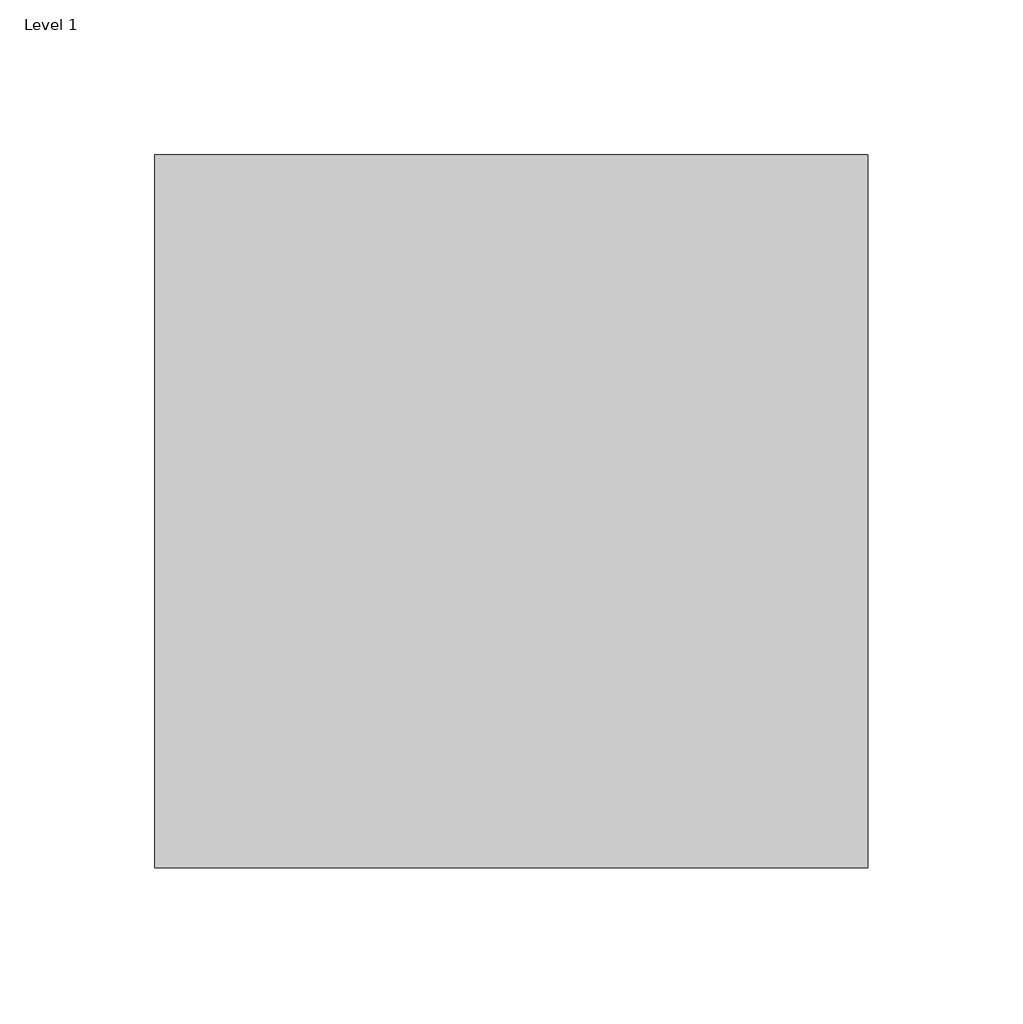
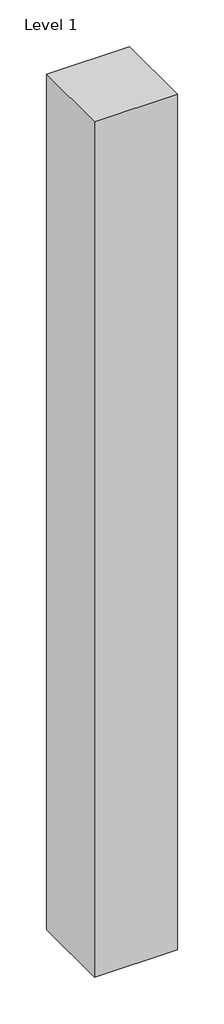
# One storey, part 1 of 2: 1 column.
"""IFC4 building model written with IfcOpenShell, lengths in millimetres."""

import ifcopenshell
import ifcopenshell.guid

model = None  # the IFC model being written
_history = None  # IfcOwnerHistory: only IFC2X3 demands one
_inside = {}  # id of a spatial element -> (the spatial element, [elements in it])
_under = {}  # id of a project, library or spatial element -> (it, [spatial elements below it])
_declared = {}  # id of a project -> (the project, [libraries it declares])
_typed = {}  # id of a type object -> (the type object, [elements of that type])
_made_of = {}  # id of a material, layer set ... -> (it, [elements and type objects made of it])


def new_model(schema):
    """Start an empty IFC model of exactly this schema.

    Asked for "IFC4X3", IfcOpenShell would pick the latest addendum, in which some entities
    have other attributes; the version numbers below select the first issue.
    IFC2X3 requires an IfcOwnerHistory on every rooted entity: one is made here for all.
    """
    global model, _history
    if schema == "IFC4X3":
        model = ifcopenshell.file(schema_version=(4, 3, 0, 0))
    else:
        model = ifcopenshell.file(schema=schema)
    _inside.clear()
    _under.clear()
    _declared.clear()
    _typed.clear()
    _made_of.clear()
    _history = None
    if model.schema == "IFC2X3":
        org = make("IfcOrganization", Name="unknown")
        user = make(
            "IfcPersonAndOrganization",
            ThePerson=make("IfcPerson", FamilyName="unknown"),
            TheOrganization=org,
        )
        app = make(
            "IfcApplication",
            ApplicationDeveloper=org,
            Version="unknown",
            ApplicationFullName="unknown",
            ApplicationIdentifier="unknown",
        )
        _history = make(
            "IfcOwnerHistory",
            OwningUser=user,
            OwningApplication=app,
            ChangeAction="ADDED",
            CreationDate=0,
        )
    return model


def make(cls, **values):
    """One entity of the class cls with the attributes given. An attribute that is None is left unset."""
    return model.create_entity(
        cls, **{name: value for name, value in values.items() if value is not None}
    )


def rooted(cls, **values):
    """An entity with a GlobalId (a new one), such as an element, a storey or a relation."""
    return make(cls, GlobalId=ifcopenshell.guid.new(), OwnerHistory=_history, **values)


def si_unit(unit_type, name, prefix=None):
    """IfcSIUnit, for example si_unit("LENGTHUNIT", "METRE", prefix="MILLI")."""
    return make("IfcSIUnit", UnitType=unit_type, Prefix=prefix, Name=name)


def assignment(units):
    """IfcUnitAssignment: the units of a project."""
    return None if units is None else make("IfcUnitAssignment", Units=units)


def point(xyz):
    """IfcCartesianPoint."""
    return None if xyz is None else make("IfcCartesianPoint", Coordinates=xyz)


def direction(xyz):
    """IfcDirection."""
    return None if xyz is None else make("IfcDirection", DirectionRatios=xyz)


def frame(location, z_axis=None, x_axis=None):
    """IfcAxis2Placement3D, a coordinate frame: its origin and axes. An axis left out is left unset."""
    return make(
        "IfcAxis2Placement3D",
        Location=point(location),
        Axis=direction(z_axis),
        RefDirection=direction(x_axis),
    )


def origin():
    """The frame at (0, 0, 0) with its axes left unset."""
    return frame((0.0, 0.0, 0.0))


def place(relative_to, where):
    """IfcLocalPlacement: puts the frame where relative to a parent placement (None: the world)."""
    return make(
        "IfcLocalPlacement", PlacementRelTo=relative_to, RelativePlacement=where
    )


def context(
    kind, dimensions, precision=None, world=None, true_north=None, identifier=None
):
    """IfcGeometricRepresentationContext, for example the 3D "Model" context."""
    return make(
        "IfcGeometricRepresentationContext",
        ContextIdentifier=identifier,
        ContextType=kind,
        CoordinateSpaceDimension=dimensions,
        Precision=precision,
        WorldCoordinateSystem=world,
        TrueNorth=true_north,
    )


def project(units=None, contexts=None):
    """IfcProject with its units and contexts."""
    return rooted(
        "IfcProject",
        Name="project",
        RepresentationContexts=contexts,
        UnitsInContext=assignment(units),
    )


def spatial(cls, under=None, at=None, **own):
    """A site, building, storey or space (cls), placed at a placement, below another one or the project."""
    s = rooted(cls, ObjectPlacement=at, **own)
    if under is not None:
        _under.setdefault(under.id(), (under, []))[1].append(s)
    return s


def polyline(points):
    """IfcPolyline through the points."""
    return make("IfcPolyline", Points=[point(p) for p in points])


def outline(outer, holes=None, kind="AREA"):
    """IfcArbitraryClosedProfileDef: a profile drawn as a closed curve; with holes, ...WithVoids."""
    if holes is None:
        return make("IfcArbitraryClosedProfileDef", ProfileType=kind, OuterCurve=outer)
    return make(
        "IfcArbitraryProfileDefWithVoids",
        ProfileType=kind,
        OuterCurve=outer,
        InnerCurves=holes,
    )


def extrude(swept, where, along, depth):
    """IfcExtrudedAreaSolid: the profile swept, set in the frame where, extruded along a direction by depth."""
    return make(
        "IfcExtrudedAreaSolid",
        SweptArea=swept,
        Position=where,
        ExtrudedDirection=direction(along),
        Depth=depth,
    )


def shape(context_of_items, identifier, shape_type, items):
    """IfcShapeRepresentation: the items that make up one representation, for example the "Body"."""
    return make(
        "IfcShapeRepresentation",
        ContextOfItems=context_of_items,
        RepresentationIdentifier=identifier,
        RepresentationType=shape_type,
        Items=items,
    )


def source(mapping_origin, context_of_items, identifier, shape_type, items):
    """IfcRepresentationMap: a shape defined once, which mapped items show again and again."""
    return make(
        "IfcRepresentationMap",
        MappingOrigin=mapping_origin,
        MappedRepresentation=shape(context_of_items, identifier, shape_type, items),
    )


def transform(
    local_origin,
    x_axis=None,
    y_axis=None,
    z_axis=None,
    scale=None,
    scale2=None,
    scale3=None,
    uniform=True,
):
    """IfcCartesianTransformationOperator3D, or its non-uniform kind. x_axis, y_axis, z_axis: its Axis1, 2, 3."""
    if uniform:
        return make(
            "IfcCartesianTransformationOperator3D",
            Axis1=direction(x_axis),
            Axis2=direction(y_axis),
            LocalOrigin=point(local_origin),
            Scale=scale,
            Axis3=direction(z_axis),
        )
    return make(
        "IfcCartesianTransformationOperator3DnonUniform",
        Axis1=direction(x_axis),
        Axis2=direction(y_axis),
        LocalOrigin=point(local_origin),
        Scale=scale,
        Axis3=direction(z_axis),
        Scale2=scale2,
        Scale3=scale3,
    )


def mapped(mapping_source, mapping_target):
    """IfcMappedItem: shows the shape of a source again, moved by a transform."""
    return make(
        "IfcMappedItem", MappingSource=mapping_source, MappingTarget=mapping_target
    )


def made_of(thing, what):
    """Note that an element or type object is made of a material, layer set ...; save() writes the relation."""
    if what is not None:
        _made_of.setdefault(what.id(), (what, []))[1].append(thing)
    return thing


def element(
    cls,
    number,
    at=None,
    inside=None,
    cuts=None,
    type_object=None,
    material=None,
    context=None,
    identifier="Body",
    shape_type=None,
    held_by="IfcProductDefinitionShape",
    body=None,
    shapes=None,
    **own,
):
    """One element of the class cls, such as IfcWall. Its Tag is "e" and its number.

    at: its placement. inside: the storey or other place that contains it. cuts: it is an
    opening in that element (IfcRelVoidsElement). A single representation is given by context,
    identifier, shape_type and body (its items); several are given by shapes. held_by: the class
    of the entity that holds the representations. save() writes the other relations.
    """
    e = rooted(cls, Tag="e%d" % number, ObjectPlacement=at, **own)
    if body is not None:
        shapes = [shape(context, identifier, shape_type, body)]
    if shapes is not None:
        e.Representation = make(held_by, Representations=shapes)
    if inside is not None:
        _inside.setdefault(inside.id(), (inside, []))[1].append(e)
    if cuts is not None:
        rooted(
            "IfcRelVoidsElement", RelatingBuildingElement=cuts, RelatedOpeningElement=e
        )
    if type_object is not None:
        _typed.setdefault(type_object.id(), (type_object, []))[1].append(e)
    return made_of(e, material)


def aggregate(whole, parts):
    """IfcRelAggregates: a whole, such as a stair, and the parts it consists of."""
    return rooted("IfcRelAggregates", RelatingObject=whole, RelatedObjects=parts)


def save(model, path):
    """Write the relations noted so far, then the file.

    IfcRelAggregates (storeys below a building ...), IfcRelContainedInSpatialStructure (elements
    in a storey), IfcRelDefinesByType, IfcRelAssociatesMaterial and IfcRelDeclares: one each for
    every whole, place, type object, material and project.
    """
    for whole, parts in _under.values():
        aggregate(whole, parts)
    for where, things in _inside.values():
        rooted(
            "IfcRelContainedInSpatialStructure",
            RelatedElements=things,
            RelatingStructure=where,
        )
    for kind, things in _typed.values():
        rooted("IfcRelDefinesByType", RelatedObjects=things, RelatingType=kind)
    for what, things in _made_of.values():
        rooted("IfcRelAssociatesMaterial", RelatedObjects=things, RelatingMaterial=what)
    for by, libraries in _declared.values():
        rooted("IfcRelDeclares", RelatingContext=by, RelatedDefinitions=libraries)
    model.write(path)


def concrete_rectangular_column_230_x230mm_2_460f90e7(model_context):
    return source(origin(), model_context, "Body", "SweptSolid", [
        extrude(outline(polyline([(115.0, 115.0), (115.0, -115.0), (-115.0, -115.0), (-115.0, 115.0), (115.0, 115.0)])), frame((0.0, 0.0, -2500.0), z_axis=(0.0, 0.0, 1.0), x_axis=(1.0, 0.0, 0.0)), (0.0, 0.0, 1.0), 2500.0),
    ])


model = new_model("IFC4")

# Units and contexts
model_context = context("Model", 3, world=origin())
ifc_project = project(units=[si_unit("LENGTHUNIT", "METRE", prefix="MILLI")], contexts=[model_context])

# Site, building, storey
site = spatial("IfcSite", under=ifc_project)
building = spatial("IfcBuilding", under=site)
storey = spatial("IfcBuildingStorey", under=building, Name="Level 1", Elevation=0.0)

# Column
placement = place(None, origin())
concrete_rectangular_column_230_x230mm_2_shape = concrete_rectangular_column_230_x230mm_2_460f90e7(model_context)
element("IfcColumn", 1, ObjectType="Concrete-Rectangular-Column : 230 x230mm 2", at=placement, inside=storey, context=model_context, shape_type="MappedRepresentation", body=[
    mapped(concrete_rectangular_column_230_x230mm_2_shape, transform((-9149.2529311, -1337.0359052, 0.0), x_axis=(1.0, 0.0, 0.0), y_axis=(0.0, 1.0, 0.0), z_axis=(0.0, 0.0, 1.0))),
])

save(model, "model.ifc")

# Revit data of these elements
# Project information
#   Project Issue Date = "Issue Date"
#   Project Status = "Project Status"
#   Client Name = "Owner"
#   Project Address = "Enter address here"
#   Project Name = "Project Name"
#   Project Number = "Project Number"
# Type "Concrete-Rectangular-Column : 230 x230mm 2"
#   b = 230 mm
#   h = 230 mm
#   Structural Material [instance default] = Concrete, Cast-in-Place gray
# Element 1 (IfcColumn, "Concrete-Rectangular-Column : 230 x230mm 2")
#   Structural Material = Concrete, Cast-in-Place gray
#   Phase Created = New Construction
#   Materials on its faces: "Concrete, Cast-in-Place gray"
# Materials
#   "Concrete, Cast-in-Place gray": class "Concrete", colour RGB 192 192 192, transparency 0, Description = "Cast-in-place concrete", Cost = 0
